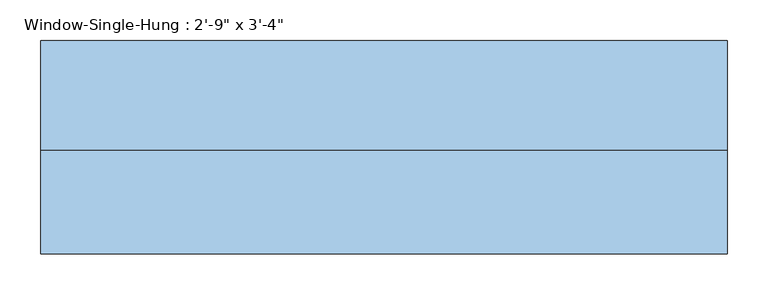
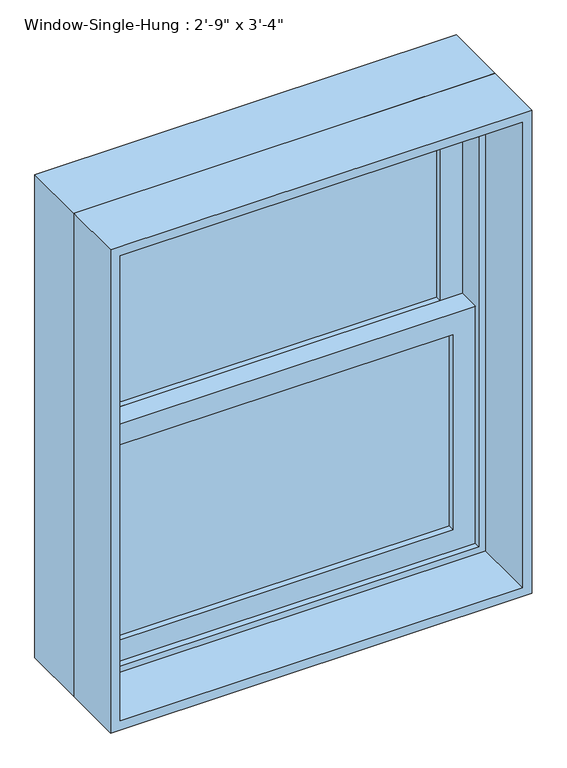
"""IFC4 building model written with IfcOpenShell, lengths in millimetres: window geometry."""

from ifc_helpers import new_model, si_unit, frame, origin, place, context, project, spatial, polyline, outline, extrude, source, transform, mapped, element, save


def window_aaa0cff3(model_context):
    return source(origin(), model_context, "Body", "SweptSolid", [
        extrude(outline(polyline([(342.9, 50.8), (342.9, 44.45), (-342.9, 44.45), (-342.9, 50.8), (342.9, 50.8)])), frame((0.0, 0.0, 990.6), z_axis=(0.0, 0.0, 1.0), x_axis=(1.0, 0.0, 0.0)), (0.0, 0.0, 1.0), 409.575),
        extrude(outline(polyline([(-342.9, 38.1), (342.9, 38.1), (342.9, 31.75), (-342.9, 31.75), (-342.9, 38.1)])), frame((0.0, 0.0, 990.6), z_axis=(0.0, 0.0, 1.0), x_axis=(1.0, 0.0, 0.0)), (0.0, 0.0, 1.0), 409.575),
        extrude(outline(polyline([(342.9, 95.25), (342.9, 88.9), (-342.9, 88.9), (-342.9, 95.25), (342.9, 95.25)])), frame((0.0, 0.0, 1444.625), z_axis=(0.0, 0.0, 1.0), x_axis=(1.0, 0.0, 0.0)), (0.0, 0.0, 1.0), 409.575),
        extrude(outline(polyline([(-342.9, 82.55), (342.9, 82.55), (342.9, 76.2), (-342.9, 76.2), (-342.9, 82.55)])), frame((0.0, 0.0, 1444.625), z_axis=(0.0, 0.0, 1.0), x_axis=(1.0, 0.0, 0.0)), (0.0, 0.0, 1.0), 409.575),
        extrude(outline(polyline([(1444.625, -387.35), (946.15, -387.35), (946.15, 387.35), (1444.625, 387.35), (1444.625, -387.35)]), holes=[polyline([(1400.175, 342.9), (990.6, 342.9), (990.6, -342.9), (1400.175, -342.9), (1400.175, 342.9)])]), frame((0.0, 19.05, 0.0), z_axis=(0.0, 1.0, 0.0), x_axis=(0.0, 0.0, 1.0)), (0.0, 0.0, 1.0), 44.45),
        extrude(outline(polyline([(1898.65, -387.35), (1400.175, -387.35), (1400.175, 387.35), (1898.65, 387.35), (1898.65, -387.35)]), holes=[polyline([(1854.2, 342.9), (1444.625, 342.9), (1444.625, -342.9), (1854.2, -342.9), (1854.2, 342.9)])]), frame((0.0, 63.5, 0.0), z_axis=(0.0, 1.0, 0.0), x_axis=(0.0, 0.0, 1.0)), (0.0, 0.0, 1.0), 44.45),
        extrude(outline(polyline([(1930.4, -419.1), (914.4, -419.1), (914.4, 419.1), (1930.4, 419.1), (1930.4, -419.1)]), holes=[polyline([(1898.65, 387.35), (946.15, 387.35), (946.15, -387.35), (1898.65, -387.35), (1898.65, 387.35)])]), frame((0.0, 6.35, 0.0), z_axis=(0.0, 1.0, 0.0), x_axis=(0.0, 0.0, 1.0)), (0.0, 0.0, 1.0), 133.35),
        extrude(outline(polyline([(1930.4, 419.1), (1930.4, -419.1), (914.4, -419.1), (914.4, 419.1), (1930.4, 419.1)]), holes=[polyline([(1911.35, 400.05), (933.45, 400.05), (933.45, -400.05), (1911.35, -400.05), (1911.35, 400.05)])]), frame((0.0, -120.65, 0.0), z_axis=(0.0, 1.0, 0.0), x_axis=(0.0, 0.0, 1.0)), (0.0, 0.0, 1.0), 127.0),
    ])


if __name__ == "__main__":
    model = new_model("IFC4")
    model_context = context("Model", 3, world=origin())
    ifc_project = project(units=[si_unit("LENGTHUNIT", "METRE", prefix="MILLI")], contexts=[model_context])
    site = spatial("IfcSite", under=ifc_project)
    building = spatial("IfcBuilding", under=site)
    placement = place(None, origin())
    window_shape = window_aaa0cff3(model_context)
    element("IfcWindow", 1, ObjectType="Window-Single-Hung : 2'-9\" x 3'-4\"", at=placement, inside=building, context=model_context, shape_type="MappedRepresentation", body=[
        mapped(window_shape, transform((0.0, 0.0, 0.0), x_axis=(1.0, 0.0, 0.0), y_axis=(0.0, 1.0, 0.0), z_axis=(0.0, 0.0, 1.0))),
    ])
    save(model, "model.ifc")

# Revit data of these elements
# Type "Window-Single-Hung : 2'-9\" x 3'-4\""
#   Type Mark = "04"
#   Fire Rating = "0.5h"
#   Construction Type Id = "DG-DR"
#   Assembly Code = "B2020100"
#   Analytic Construction = "Double glazing - domestic"
#   Wall Thickness [instance default] = 0' - 6"
#   Window Inset [instance default] = 0' - 0"
#   Visual Light Transmittance = 0.81
#   Thermal Resistance (R) = 0.319569 (m²·K)/W
#   Solar Heat Gain Coefficient = 0.76
#   Muntin Width = 2' - 3"
#   Muntin Height = 1' - 4 1/8"
#   Interior Wall Closure [instance default] = 0' - 1 1/2"
#   Rough Width = 2' - 9 1/2"
#   Rough Height = 3' - 4 1/2"
#   Frame Extension [instance default] = 0' - 1 1/4"
#   Exterior Wall Closure [instance default] = 0' - 0 1/2"
#   Extension Jamb [instance default] = 0' - 1 1/2"
#   Heat Transfer Coefficient (U) = 3.12929 W/(m²·K)
#   Height = 3' - 4"
#   Width = 2' - 9"
#   Top Muntin Visibility = no
#   Indicator Visibility = no
#   Extension Jamb Visibility [instance default] = yes
#   Interior Trim Visibility [instance default] = yes
#   Exterior Trim Visibility [instance default] = yes
#   Bottom Muntin Visibility = no
#   Muntin Pattern = Muntin Pattern_2x2 : Muntin Pattern_2x2
#   Interior Trim Material = 1X WOOD COMPOSITE TRIM
#   Interior Trim = Trim-Window-Interior-Flat : Picture Frame
#   Exterior Trim Material = 1X WOOD COMPOSITE TRIM
#   Exterior Trim = Trim-Window-Exterior-Flat : with Sill
#   Glass Panel Material = NEW DOUBLE HUNG WINDOWS (TYP.)
#   Exterior Frame Material = 1X WOOD COMPOSITE TRIM
#   Interior Frame Material = 1X WOOD COMPOSITE TRIM
#   Wall Closure = (empty or 0)
# Element 1 (IfcWindow, "Window-Single-Hung : 2'-9\" x 3'-4\"")
#   Wall Thickness = 0' - 9 1/2"
#   Extension Jamb = 0' - 5"
#   Materials on its faces: "1X WOOD COMPOSITE TRIM", "NEW DOUBLE HUNG WINDOWS (TYP.)"
# Materials
#   "1X WOOD COMPOSITE TRIM": class "Generic", colour RGB 88 61 61, transparency 0, Cost = 0
#   "NEW DOUBLE HUNG WINDOWS (TYP.)": class "Glass", colour RGB 218 227 224, transparency 0.85, Description = "Soda Lime Glass", Cost = 0
